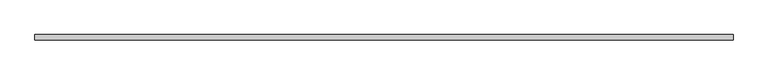
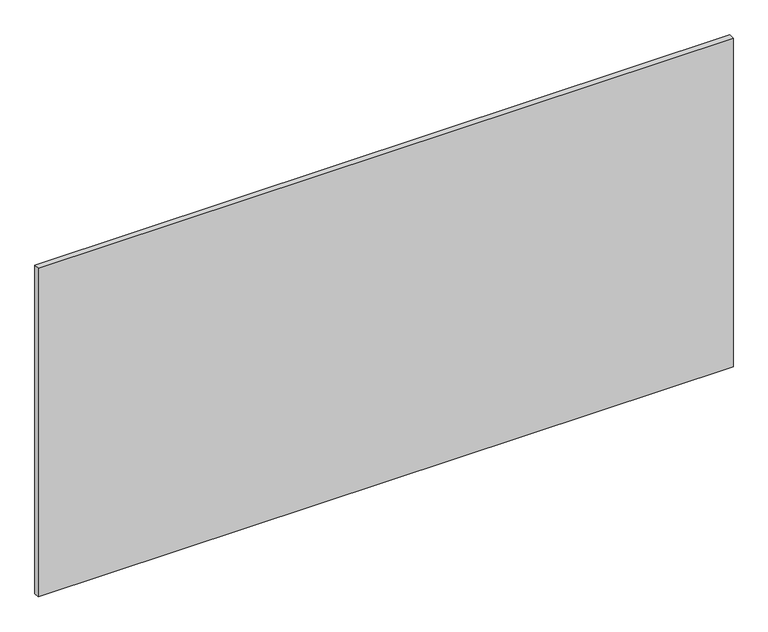
"""IFC4 building model written with IfcOpenShell, lengths in millimetres: proxy geometry, Inner panel:Inner panel:1:Inner panel:1 : Inner panel:Inner panel:300324:300043:Inner panel:1:Inner panel:1 : Inner panel:Inner panel:300324:300043 : Inner panel:Inner panel:1:Inner panel:1 : Inner panel:Inner panel:300324:300043:14 : Inner panel:Inner panel:1:Inner panel:1 : Inner panel:Inner panel:300324:300043:Inner panel:1:Inner panel:1 : Inner panel:Inner panel:300324:300043 : Inner panel:Inner panel:1:Inner panel:1 : Inner panel:Inner panel:300324:300043:300031."""

from ifc_helpers import new_model, si_unit, frame, origin, place, context, project, spatial, polyline, outline, extrude, source, transform, mapped, element, save


def generic_models_a8e4db55(model_context):
    return source(origin(), model_context, "Body", "SweptSolid", [
        extrude(outline(polyline([(570452.6367239, -578778.4413841), (572891.0367239, -578778.4413841), (572891.0367239, -578797.4913841), (570452.6367239, -578797.4913841), (570452.6367239, -578778.4413841)])), frame((0.0, 0.0, 44.45), z_axis=(0.0, 0.0, 1.0), x_axis=(1.0, 0.0, 0.0)), (0.0, 0.0, 1.0), 1219.2),
    ])


if __name__ == "__main__":
    model = new_model("IFC4")
    model_context = context("Model", 3, world=origin())
    ifc_project = project(units=[si_unit("LENGTHUNIT", "METRE", prefix="MILLI")], contexts=[model_context])
    site = spatial("IfcSite", under=ifc_project)
    building = spatial("IfcBuilding", under=site)
    placement = place(None, origin())
    generic_models_shape = generic_models_a8e4db55(model_context)
    element("IfcBuildingElementProxy", 1, Name="Inner panel:Inner panel:1:Inner panel:1 : Inner panel:Inner panel:300324:300043:Inner panel:1:Inner panel:1 : Inner panel:Inner panel:300324:300043 : Inner panel:Inner panel:1:Inner panel:1 : Inner panel:Inner panel:300324:300043:14 : Inner panel:Inner panel:1:Inner panel:1 : Inner panel:Inner panel:300324:300043:Inner panel:1:Inner panel:1 : Inner panel:Inner panel:300324:300043 : Inner panel:Inner panel:1:Inner panel:1 : Inner panel:Inner panel:300324:300043:300031", ObjectType="Inner panel:Inner panel:1:Inner panel:1 : Inner panel:Inner panel:300324:300043:Inner panel:1:Inner panel:1 : Inner panel:Inner panel:300324:300043 : Inner panel:Inner panel:1:Inner panel:1 : Inner panel:Inner panel:300324:300043:14 : Inner panel:Inner panel:1:Inner panel:1 : Inner panel:Inner panel:300324:300043:Inner panel:1:Inner panel:1 : Inner panel:Inner panel:300324:300043 : Inner panel:Inner panel:1:Inner panel:1 : Inner panel:Inner panel:300324:300043:300031", at=placement, inside=building, context=model_context, shape_type="MappedRepresentation", body=[
        mapped(generic_models_shape, transform((0.0, 0.0, 0.0), x_axis=(1.0, 0.0, 0.0), y_axis=(0.0, 1.0, 0.0), z_axis=(0.0, 0.0, 1.0))),
    ])
    save(model, "model.ifc")

# Revit data of these elements
# Type "Inner panel:Inner panel:1:Inner panel:1 : Inner panel:Inner panel:300324:300043:Inner panel:1:Inner panel:1 : Inner panel:Inner panel:300324:300043 : Inner panel:Inner panel:1:Inner panel:1 : Inner panel:Inner panel:300324:300043:14 : Inner panel:Inner panel:1:Inner panel:1 : Inner panel:Inner panel:300324:300043:Inner panel:1:Inner panel:1 : Inner panel:Inner panel:300324:300043 : Inner panel:Inner panel:1:Inner panel:1 : Inner panel:Inner panel:300324:300043:300031"
#   NameOverride = "Inner panel:Inner panel:1:Inner panel:1 : Inner panel:Inner panel:300324:300043:Inner panel:1:Inner panel:1 : Inner panel:Inner panel:300324:300043 : Inner panel:Inner panel:1:Inner panel:1 : Inner panel:Inner panel:300324:300043:300031"
#   ObjectTypeOverride = "Inner panel:1:Inner panel:1 : Inner panel:Inner panel:300324:300043 : Inner panel:Inner panel:1:Inner panel:1 : Inner panel:Inner panel:300324:300043"
#   Reference = "Inner panel"
#   Tag = "300031"
# Element 1 (IfcBuildingElementProxy, "Inner panel:Inner panel:1:Inner panel:1 : Inner panel:Inner panel:300324:300043:Inner panel:1:Inner panel:1 : Inner panel:Inner panel:300324:300043 : Inner panel:Inner panel:1:Inner panel:1 : Inner panel:Inner panel:300324:300043:14 : Inner panel:Inner panel:1:Inner panel:1 : Inner panel:Inner panel:300324:300043:Inner panel:1:Inner panel:1 : Inner panel:Inner panel:300324:300043 : Inner panel:Inner panel:1:Inner panel:1 : Inner panel:Inner panel:300324:300043:300031")
#   Materials on its faces: "¾” (CLASS A) FIRE RETARDANT PLYWOOD ...OR… IF 1/4\" GYP. BD UNDER PLYWOOD, FLAME SPREAD TO BE CLASS C -  (FINISH: GRADE B - PREFINISHED STAINED/SEALED) - 1/4\" GAP BTWN PANELS (FASTENERS T.B.D.)"
# Materials
#   "¾” (CLASS A) FIRE RETARDANT PLYWOOD ...OR… IF 1/4\" GYP. BD UNDER PLYWOOD, FLAME SPREAD TO BE CLASS C -  (FINISH: GRADE B - PREFINISHED STAINED/SEALED) - 1/4\" GAP BTWN PANELS (FASTENERS T.B.D.)": class "Wood", colour RGB 149 120 74, transparency 0, Description = "Plywood, sheathing grade", Cost = 0
